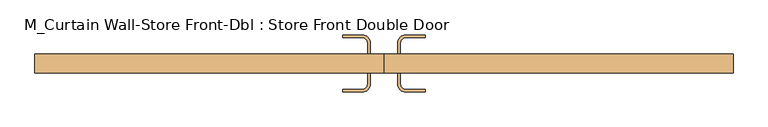
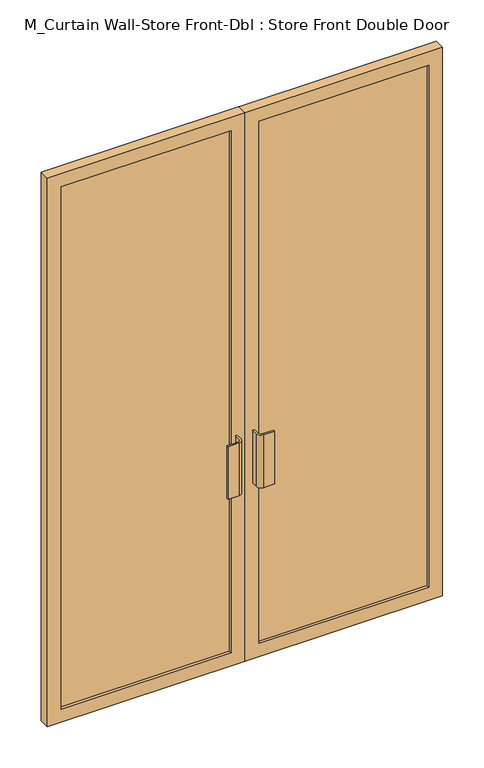
"""IFC4 building model written with IfcOpenShell, lengths in millimetres: door geometry, M_Curtain Wall-Store Front-Dbl : Store Front Double Door."""

import ifcopenshell
import ifcopenshell.guid

model = None  # the IFC model being written
_history = None  # IfcOwnerHistory: only IFC2X3 demands one
_inside = {}  # id of a spatial element -> (the spatial element, [elements in it])
_under = {}  # id of a project, library or spatial element -> (it, [spatial elements below it])
_declared = {}  # id of a project -> (the project, [libraries it declares])
_typed = {}  # id of a type object -> (the type object, [elements of that type])
_made_of = {}  # id of a material, layer set ... -> (it, [elements and type objects made of it])


def new_model(schema):
    """Start an empty IFC model of exactly this schema.

    Asked for "IFC4X3", IfcOpenShell would pick the latest addendum, in which some entities
    have other attributes; the version numbers below select the first issue.
    IFC2X3 requires an IfcOwnerHistory on every rooted entity: one is made here for all.
    """
    global model, _history
    if schema == "IFC4X3":
        model = ifcopenshell.file(schema_version=(4, 3, 0, 0))
    else:
        model = ifcopenshell.file(schema=schema)
    _inside.clear()
    _under.clear()
    _declared.clear()
    _typed.clear()
    _made_of.clear()
    _history = None
    if model.schema == "IFC2X3":
        org = make("IfcOrganization", Name="unknown")
        user = make(
            "IfcPersonAndOrganization",
            ThePerson=make("IfcPerson", FamilyName="unknown"),
            TheOrganization=org,
        )
        app = make(
            "IfcApplication",
            ApplicationDeveloper=org,
            Version="unknown",
            ApplicationFullName="unknown",
            ApplicationIdentifier="unknown",
        )
        _history = make(
            "IfcOwnerHistory",
            OwningUser=user,
            OwningApplication=app,
            ChangeAction="ADDED",
            CreationDate=0,
        )
    return model


def make(cls, **values):
    """One entity of the class cls with the attributes given. An attribute that is None is left unset."""
    return model.create_entity(
        cls, **{name: value for name, value in values.items() if value is not None}
    )


def rooted(cls, **values):
    """An entity with a GlobalId (a new one), such as an element, a storey or a relation."""
    return make(cls, GlobalId=ifcopenshell.guid.new(), OwnerHistory=_history, **values)


def si_unit(unit_type, name, prefix=None):
    """IfcSIUnit, for example si_unit("LENGTHUNIT", "METRE", prefix="MILLI")."""
    return make("IfcSIUnit", UnitType=unit_type, Prefix=prefix, Name=name)


def assignment(units):
    """IfcUnitAssignment: the units of a project."""
    return None if units is None else make("IfcUnitAssignment", Units=units)


def point(xyz):
    """IfcCartesianPoint."""
    return None if xyz is None else make("IfcCartesianPoint", Coordinates=xyz)


def direction(xyz):
    """IfcDirection."""
    return None if xyz is None else make("IfcDirection", DirectionRatios=xyz)


def frame(location, z_axis=None, x_axis=None):
    """IfcAxis2Placement3D, a coordinate frame: its origin and axes. An axis left out is left unset."""
    return make(
        "IfcAxis2Placement3D",
        Location=point(location),
        Axis=direction(z_axis),
        RefDirection=direction(x_axis),
    )


def frame_2d(location, x_axis=None):
    """IfcAxis2Placement2D, a coordinate frame in the plane: its origin and x axis."""
    return make(
        "IfcAxis2Placement2D", Location=point(location), RefDirection=direction(x_axis)
    )


def origin():
    """The frame at (0, 0, 0) with its axes left unset."""
    return frame((0.0, 0.0, 0.0))


def place(relative_to, where):
    """IfcLocalPlacement: puts the frame where relative to a parent placement (None: the world)."""
    return make(
        "IfcLocalPlacement", PlacementRelTo=relative_to, RelativePlacement=where
    )


def context(
    kind, dimensions, precision=None, world=None, true_north=None, identifier=None
):
    """IfcGeometricRepresentationContext, for example the 3D "Model" context."""
    return make(
        "IfcGeometricRepresentationContext",
        ContextIdentifier=identifier,
        ContextType=kind,
        CoordinateSpaceDimension=dimensions,
        Precision=precision,
        WorldCoordinateSystem=world,
        TrueNorth=true_north,
    )


def project(units=None, contexts=None):
    """IfcProject with its units and contexts."""
    return rooted(
        "IfcProject",
        Name="project",
        RepresentationContexts=contexts,
        UnitsInContext=assignment(units),
    )


def spatial(cls, under=None, at=None, **own):
    """A site, building, storey or space (cls), placed at a placement, below another one or the project."""
    s = rooted(cls, ObjectPlacement=at, **own)
    if under is not None:
        _under.setdefault(under.id(), (under, []))[1].append(s)
    return s


def polyline(points):
    """IfcPolyline through the points."""
    return make("IfcPolyline", Points=[point(p) for p in points])


def circle_curve(where, radius):
    """IfcCircle in the frame where."""
    return make("IfcCircle", Position=where, Radius=radius)


def trimmed(basis, trim1, trim2, sense, master):
    """IfcTrimmedCurve: the piece of a basis curve between two trims."""
    return make(
        "IfcTrimmedCurve",
        BasisCurve=basis,
        Trim1=trim1,
        Trim2=trim2,
        SenseAgreement=sense,
        MasterRepresentation=master,
    )


def segment(curve, same_sense, transition):
    """IfcCompositeCurveSegment."""
    return make(
        "IfcCompositeCurveSegment",
        Transition=transition,
        SameSense=same_sense,
        ParentCurve=curve,
    )


def composite_curve(segments, self_intersect=None):
    """IfcCompositeCurve: segments joined end to end."""
    return make("IfcCompositeCurve", Segments=segments, SelfIntersect=self_intersect)


def outline(outer, holes=None, kind="AREA"):
    """IfcArbitraryClosedProfileDef: a profile drawn as a closed curve; with holes, ...WithVoids."""
    if holes is None:
        return make("IfcArbitraryClosedProfileDef", ProfileType=kind, OuterCurve=outer)
    return make(
        "IfcArbitraryProfileDefWithVoids",
        ProfileType=kind,
        OuterCurve=outer,
        InnerCurves=holes,
    )


def extrude(swept, where, along, depth):
    """IfcExtrudedAreaSolid: the profile swept, set in the frame where, extruded along a direction by depth."""
    return make(
        "IfcExtrudedAreaSolid",
        SweptArea=swept,
        Position=where,
        ExtrudedDirection=direction(along),
        Depth=depth,
    )


def shape(context_of_items, identifier, shape_type, items):
    """IfcShapeRepresentation: the items that make up one representation, for example the "Body"."""
    return make(
        "IfcShapeRepresentation",
        ContextOfItems=context_of_items,
        RepresentationIdentifier=identifier,
        RepresentationType=shape_type,
        Items=items,
    )


def source(mapping_origin, context_of_items, identifier, shape_type, items):
    """IfcRepresentationMap: a shape defined once, which mapped items show again and again."""
    return make(
        "IfcRepresentationMap",
        MappingOrigin=mapping_origin,
        MappedRepresentation=shape(context_of_items, identifier, shape_type, items),
    )


def transform(
    local_origin,
    x_axis=None,
    y_axis=None,
    z_axis=None,
    scale=None,
    scale2=None,
    scale3=None,
    uniform=True,
):
    """IfcCartesianTransformationOperator3D, or its non-uniform kind. x_axis, y_axis, z_axis: its Axis1, 2, 3."""
    if uniform:
        return make(
            "IfcCartesianTransformationOperator3D",
            Axis1=direction(x_axis),
            Axis2=direction(y_axis),
            LocalOrigin=point(local_origin),
            Scale=scale,
            Axis3=direction(z_axis),
        )
    return make(
        "IfcCartesianTransformationOperator3DnonUniform",
        Axis1=direction(x_axis),
        Axis2=direction(y_axis),
        LocalOrigin=point(local_origin),
        Scale=scale,
        Axis3=direction(z_axis),
        Scale2=scale2,
        Scale3=scale3,
    )


def mapped(mapping_source, mapping_target):
    """IfcMappedItem: shows the shape of a source again, moved by a transform."""
    return make(
        "IfcMappedItem", MappingSource=mapping_source, MappingTarget=mapping_target
    )


def made_of(thing, what):
    """Note that an element or type object is made of a material, layer set ...; save() writes the relation."""
    if what is not None:
        _made_of.setdefault(what.id(), (what, []))[1].append(thing)
    return thing


def element(
    cls,
    number,
    at=None,
    inside=None,
    cuts=None,
    type_object=None,
    material=None,
    context=None,
    identifier="Body",
    shape_type=None,
    held_by="IfcProductDefinitionShape",
    body=None,
    shapes=None,
    **own,
):
    """One element of the class cls, such as IfcWall. Its Tag is "e" and its number.

    at: its placement. inside: the storey or other place that contains it. cuts: it is an
    opening in that element (IfcRelVoidsElement). A single representation is given by context,
    identifier, shape_type and body (its items); several are given by shapes. held_by: the class
    of the entity that holds the representations. save() writes the other relations.
    """
    e = rooted(cls, Tag="e%d" % number, ObjectPlacement=at, **own)
    if body is not None:
        shapes = [shape(context, identifier, shape_type, body)]
    if shapes is not None:
        e.Representation = make(held_by, Representations=shapes)
    if inside is not None:
        _inside.setdefault(inside.id(), (inside, []))[1].append(e)
    if cuts is not None:
        rooted(
            "IfcRelVoidsElement", RelatingBuildingElement=cuts, RelatedOpeningElement=e
        )
    if type_object is not None:
        _typed.setdefault(type_object.id(), (type_object, []))[1].append(e)
    return made_of(e, material)


def aggregate(whole, parts):
    """IfcRelAggregates: a whole, such as a stair, and the parts it consists of."""
    return rooted("IfcRelAggregates", RelatingObject=whole, RelatedObjects=parts)


def save(model, path):
    """Write the relations noted so far, then the file.

    IfcRelAggregates (storeys below a building ...), IfcRelContainedInSpatialStructure (elements
    in a storey), IfcRelDefinesByType, IfcRelAssociatesMaterial and IfcRelDeclares: one each for
    every whole, place, type object, material and project.
    """
    for whole, parts in _under.values():
        aggregate(whole, parts)
    for where, things in _inside.values():
        rooted(
            "IfcRelContainedInSpatialStructure",
            RelatedElements=things,
            RelatingStructure=where,
        )
    for kind, things in _typed.values():
        rooted("IfcRelDefinesByType", RelatedObjects=things, RelatingType=kind)
    for what, things in _made_of.values():
        rooted("IfcRelAssociatesMaterial", RelatedObjects=things, RelatingMaterial=what)
    for by, libraries in _declared.values():
        rooted("IfcRelDeclares", RelatingContext=by, RelatedDefinitions=libraries)
    model.write(path)


def m_curtain_wall_store_front_dbl_store_front_double_door_f57a5871(model_context):
    return source(origin(), model_context, "Body", "SweptSolid", [
        extrude(outline(composite_curve([segment(trimmed(circle_curve(frame_2d((-50.8, -14.85)), 19.05), [point((-31.75, -14.85))], [point((-50.8, -33.9))], False, "CARTESIAN"), True, "CONTINUOUS"), segment(polyline([(-50.8, -33.9), (-95.25, -33.9), (-95.25, -27.55), (-50.8, -27.55)]), True, "CONTINUOUS"), segment(trimmed(circle_curve(frame_2d((-50.8, -14.85)), 12.7), [point((-50.8, -27.55))], [point((-38.1, -14.85))], True, "CARTESIAN"), True, "CONTINUOUS"), segment(polyline([(-38.1, -14.85), (-38.1, 10.55), (-31.75, 10.55), (-31.75, -14.85)]), True, "CONTINUOUS")], self_intersect=False)), frame((0.0, 0.0, 762.0), z_axis=(0.0, 0.0, 1.0), x_axis=(1.0, 0.0, 0.0)), (0.0, 0.0, 1.0), 228.6),
        extrude(outline(composite_curve([segment(polyline([(31.75, -14.85), (31.75, 10.55), (38.1, 10.55), (38.1, -14.85)]), True, "CONTINUOUS"), segment(trimmed(circle_curve(frame_2d((50.8, -14.85)), 12.7), [point((38.1, -14.85))], [point((50.8, -27.55))], True, "CARTESIAN"), True, "CONTINUOUS"), segment(polyline([(50.8, -27.55), (95.25, -27.55), (95.25, -33.9), (50.8, -33.9)]), True, "CONTINUOUS"), segment(trimmed(circle_curve(frame_2d((50.8, -14.85)), 19.05), [point((50.8, -33.9))], [point((31.75, -14.85))], False, "CARTESIAN"), True, "CONTINUOUS")], self_intersect=False)), frame((0.0, 0.0, 762.0), z_axis=(0.0, 0.0, 1.0), x_axis=(1.0, 0.0, 0.0)), (0.0, 0.0, 1.0), 228.6),
        extrude(outline(composite_curve([segment(polyline([(-31.75, 80.4), (-31.75, 55.0), (-38.1, 55.0), (-38.1, 80.4)]), True, "CONTINUOUS"), segment(trimmed(circle_curve(frame_2d((-50.8, 80.4)), 12.7), [point((-38.1, 80.4))], [point((-50.8, 93.1))], True, "CARTESIAN"), True, "CONTINUOUS"), segment(polyline([(-50.8, 93.1), (-95.25, 93.1), (-95.25, 99.45), (-50.8, 99.45)]), True, "CONTINUOUS"), segment(trimmed(circle_curve(frame_2d((-50.8, 80.4)), 19.05), [point((-50.8, 99.45))], [point((-31.75, 80.4))], False, "CARTESIAN"), True, "CONTINUOUS")], self_intersect=False)), frame((0.0, 0.0, 762.0), z_axis=(0.0, 0.0, 1.0), x_axis=(1.0, 0.0, 0.0)), (0.0, 0.0, 1.0), 228.6),
        extrude(outline(composite_curve([segment(trimmed(circle_curve(frame_2d((50.8, 80.4)), 19.05), [point((31.75, 80.4))], [point((50.8, 99.45))], False, "CARTESIAN"), True, "CONTINUOUS"), segment(polyline([(50.8, 99.45), (95.25, 99.45), (95.25, 93.1), (50.8, 93.1)]), True, "CONTINUOUS"), segment(trimmed(circle_curve(frame_2d((50.8, 80.4)), 12.7), [point((50.8, 93.1))], [point((38.1, 80.4))], True, "CARTESIAN"), True, "CONTINUOUS"), segment(polyline([(38.1, 80.4), (38.1, 55.0), (31.75, 55.0), (31.75, 80.4)]), True, "CONTINUOUS")], self_intersect=False)), frame((0.0, 0.0, 762.0), z_axis=(0.0, 0.0, 1.0), x_axis=(1.0, 0.0, 0.0)), (0.0, 0.0, 1.0), 228.6),
        extrude(outline(polyline([(752.85, 23.25), (57.94375, 23.25), (57.94375, 42.3), (752.85, 42.3), (752.85, 23.25)])), frame((0.0, 0.0, 57.15), z_axis=(0.0, 0.0, 1.0), x_axis=(1.0, 0.0, 0.0)), (0.0, 0.0, 1.0), 2260.7),
        extrude(outline(polyline([(-57.94375, 23.25), (-752.85, 23.25), (-752.85, 42.3), (-57.94375, 42.3), (-57.94375, 23.25)])), frame((0.0, 0.0, 57.15), z_axis=(0.0, 0.0, 1.0), x_axis=(1.0, 0.0, 0.0)), (0.0, 0.0, 1.0), 2260.7),
        extrude(outline(polyline([(2375.0, 0.79375), (0.0, 0.79375), (0.0, 810.0), (2375.0, 810.0), (2375.0, 0.79375)]), holes=[polyline([(2317.85, 57.94375), (2317.85, 752.85), (57.15, 752.85), (57.15, 57.94375), (2317.85, 57.94375)])]), frame((0.0, 10.55, 0.0), z_axis=(0.0, 1.0, 0.0), x_axis=(0.0, 0.0, 1.0)), (0.0, 0.0, 1.0), 44.45),
        extrude(outline(polyline([(2375.0, -0.79375), (2375.0, -810.0), (0.0, -810.0), (0.0, -0.79375), (2375.0, -0.79375)]), holes=[polyline([(2317.85, -752.85), (2317.85, -57.94375), (57.15, -57.94375), (57.15, -752.85), (2317.85, -752.85)])]), frame((0.0, 10.55, 0.0), z_axis=(0.0, 1.0, 0.0), x_axis=(0.0, 0.0, 1.0)), (0.0, 0.0, 1.0), 44.45),
    ])


if __name__ == "__main__":
    model = new_model("IFC4")
    model_context = context("Model", 3, world=origin())
    ifc_project = project(units=[si_unit("LENGTHUNIT", "METRE", prefix="MILLI")], contexts=[model_context])
    site = spatial("IfcSite", under=ifc_project)
    building = spatial("IfcBuilding", under=site)
    placement = place(None, origin())
    m_curtain_wall_store_front_dbl_store_front_double_door_shape = m_curtain_wall_store_front_dbl_store_front_double_door_f57a5871(model_context)
    element("IfcDoor", 1, ObjectType="M_Curtain Wall-Store Front-Dbl : Store Front Double Door", at=placement, inside=building, context=model_context, shape_type="MappedRepresentation", body=[
        mapped(m_curtain_wall_store_front_dbl_store_front_double_door_shape, transform((0.0, 0.0, 0.0), x_axis=(1.0, 0.0, 0.0), y_axis=(0.0, 1.0, 0.0), z_axis=(0.0, 0.0, 1.0))),
    ])
    save(model, "model.ifc")

# Revit data of these elements
# Type "M_Curtain Wall-Store Front-Dbl : Store Front Double Door"
#   Type Mark = "33"
#   Offset = 55 mm
#   Function = 1
#   Material = Metal - Aluminum
#   Glazing Material = Glass
#   Assembly Code = ""
# Element 1 (IfcDoor, "M_Curtain Wall-Store Front-Dbl : Store Front Double Door")
#   Materials on its faces: "Metal - Aluminum", "Glass"
# Materials
#   "Metal - Aluminum": class "Metal", colour RGB 247 247 247, transparency 0
#   "Glass": class "Glass", colour RGB 0 128 192, transparency 0.9
